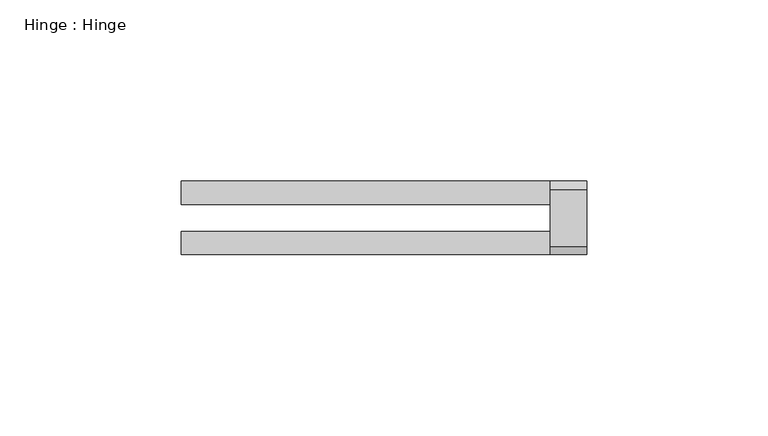
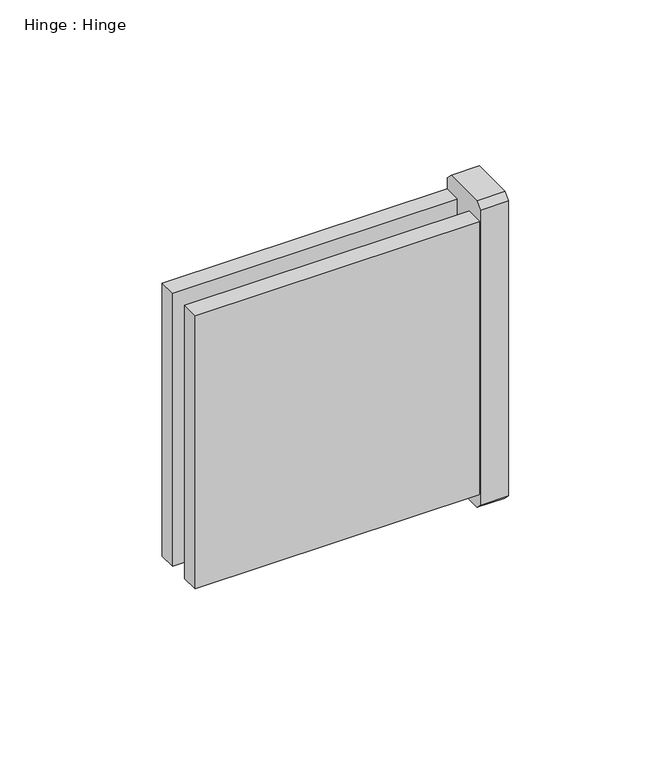
"""IFC4 building model written with IfcOpenShell, lengths in millimetres: proxy geometry, Hinge : Hinge."""

from ifc_helpers import new_model, si_unit, frame, origin, place, context, project, spatial, polyline, outline, extrude, source, transform, mapped, element, save


def hinge_hinge_cdefbeb7(model_context):
    return source(origin(), model_context, "Body", "SweptSolid", [
        extrude(outline(polyline([(9646.679882, 39394.6012561), (9630.9579547, 39394.6012561), (9628.7124545, 39396.8467563), (9628.7124545, 39507.7452438), (9630.9579547, 39509.9907439), (9646.679882, 39509.9907439), (9648.924946, 39507.7456799), (9648.924946, 39396.8463201), (9646.679882, 39394.6012561)])), frame((-9232.0719278, 0.0, 0.0), z_axis=(1.0, 0.0, 0.0), x_axis=(0.0, 1.0, 0.0)), (0.0, 0.0, 1.0), 10.0),
        extrude(outline(polyline([(-9333.6719278, 9642.574946), (-9333.6719278, 9648.924946), (-9232.0719278, 9648.924946), (-9232.0719278, 9642.574946), (-9333.6719278, 9642.574946)])), frame((0.0, 0.0, 39400.9512561), z_axis=(0.0, 0.0, 1.0), x_axis=(1.0, 0.0, 0.0)), (0.0, 0.0, 1.0), 102.6894878),
        extrude(outline(polyline([(-9333.6719278, 9628.7124545), (-9333.6719278, 9635.0624545), (-9232.0719278, 9635.0624545), (-9232.0719278, 9628.7124545), (-9333.6719278, 9628.7124545)])), frame((0.0, 0.0, 39400.9512561), z_axis=(0.0, 0.0, 1.0), x_axis=(1.0, 0.0, 0.0)), (0.0, 0.0, 1.0), 102.6894878),
    ])


if __name__ == "__main__":
    model = new_model("IFC4")
    model_context = context("Model", 3, world=origin())
    ifc_project = project(units=[si_unit("LENGTHUNIT", "METRE", prefix="MILLI")], contexts=[model_context])
    site = spatial("IfcSite", under=ifc_project)
    building = spatial("IfcBuilding", under=site)
    placement = place(None, origin())
    hinge_hinge_shape = hinge_hinge_cdefbeb7(model_context)
    element("IfcBuildingElementProxy", 1, Name="Hinge : Hinge", ObjectType="Hinge : Hinge", at=placement, inside=building, context=model_context, shape_type="MappedRepresentation", body=[
        mapped(hinge_hinge_shape, transform((0.0, 0.0, 0.0), x_axis=(1.0, 0.0, 0.0), y_axis=(0.0, 1.0, 0.0), z_axis=(0.0, 0.0, 1.0))),
    ])
    save(model, "model.ifc")

# Revit data of these elements
# Type "Hinge : Hinge"
#   NameOverride = "Hinge"
# Element 1 (IfcBuildingElementProxy, "Hinge : Hinge")
#   Materials on its faces: "HEAVY DUTY STAINLESS STEEL HINGE (90 DEGREE ROTATION)"
# Materials
#   "HEAVY DUTY STAINLESS STEEL HINGE (90 DEGREE ROTATION)": class "Unassigned", colour RGB 128 128 128, transparency 0
